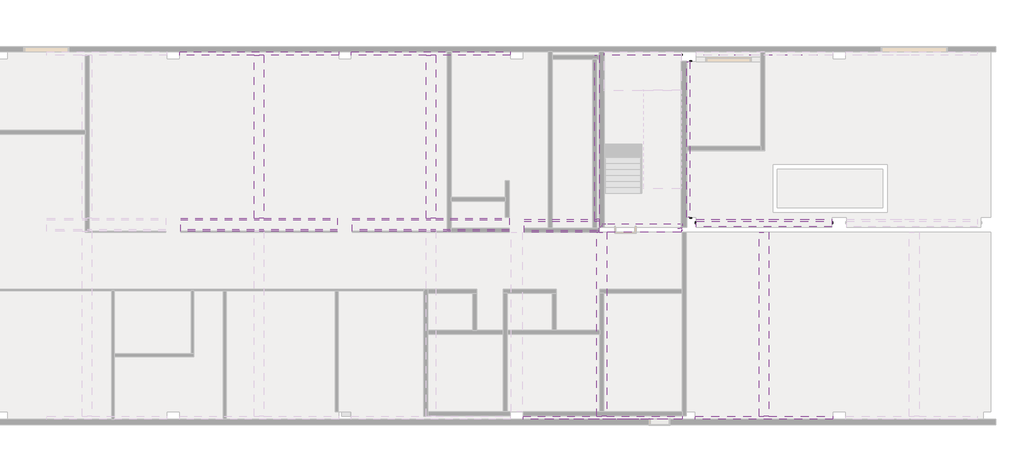
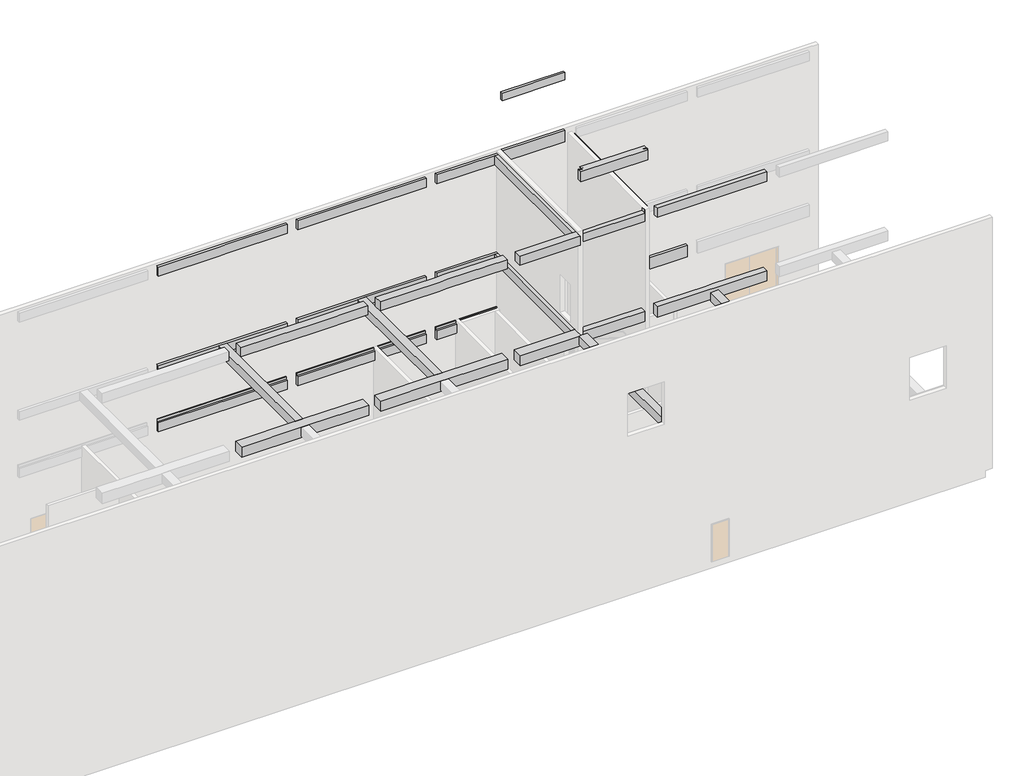
# One storey, part 4 of 5: 55 beams.
"""IFC4 building model written with IfcOpenShell, lengths in millimetres."""

from ifc_helpers import new_model, si_unit, frame, origin, place, context, project, spatial, polyline, outline, extrude, faceted_brep, element, save

model = new_model("IFC4")

# Units and contexts
model_context = context("Model", 3, world=origin())
ifc_project = project(units=[si_unit("LENGTHUNIT", "METRE", prefix="MILLI")], contexts=[model_context])

# Site, building, storey
site = spatial("IfcSite", under=ifc_project)
building = spatial("IfcBuilding", under=site)
storey = spatial("IfcBuildingStorey", under=building, Name="TOC", Elevation=149.9618634)

# Beams
placement = place(None, origin())
element("IfcBeam", 1, ObjectType="RC Beam_Rectangular : H_SB_AR_S16_UG_B500xH700_1G1", at=placement, inside=storey, context=model_context, shape_type="Brep", body=[
    faceted_brep([(61750.0, 799.5208589, -0.0381366), (61750.0, 9149.5208589, -0.0381366), (61750.0, 9149.5208589, -150.0381366), (61750.0, 9149.5208589, -550.0381366), (61750.0, 799.5208589, -550.0381366), (62250.0, 9149.5208589, -550.0381366), (62250.0, 799.5208589, -550.0381366), (62250.0, 9149.5208589, -0.0381366), (62250.0, 799.5208589, -0.0381366), (62250.0, 9149.5208589, -150.0381366)], [[[0, 1, 2, 3, 4]], [[3, 5, 6, 4]], [[7, 8, 6, 5, 9]], [[1, 0, 8, 7]], [[5, 3, 2, 1, 7, 9]], [[4, 6, 8, 0]]]),
])
element("IfcBeam", 2, ObjectType="RC Beam_Rectangular : H_SB_AR_S16_UG_B500xH700_1G1", at=placement, inside=storey, context=model_context, shape_type="Brep", body=[
    faceted_brep([(54700.0, 799.5208589, -0.0381366), (54700.0, 9149.5208589, -0.0381366), (54700.0, 9149.5208589, -150.0381366), (54700.0, 9149.5208589, -550.0381366), (54700.0, 799.5208589, -550.0381366), (54700.0, 799.5208589, -150.0381366), (55200.0, 799.5208589, -550.0381366), (54850.0, 9149.5208589, -550.0381366), (55200.0, 9149.5208589, -550.0381366), (55200.0, 9149.5208589, -0.0381366), (55200.0, 799.5208589, -0.0381366), (55200.0, 9149.5208589, -150.0381366)], [[[0, 1, 2, 3, 4, 5]], [[6, 4, 3, 7, 8]], [[9, 10, 6, 8, 11]], [[1, 0, 10, 9]], [[1, 9, 11, 8, 7, 3, 2]], [[4, 6, 10, 0, 5]]]),
])
element("IfcBeam", 3, ObjectType="RC Beam_Rectangular : H_SB_AR_S16_UG_B450xH700_1B2", at=placement, inside=storey, context=model_context, shape_type="SweptSolid", body=[
    extrude(outline(polyline([(57725.0, 599.5208589), (57275.0, 599.5208589), (57275.0, 9149.5208589), (57725.0, 9149.5208589), (57725.0, 599.5208589)])), frame((0.0, 0.0, -550.0381366), z_axis=(0.0, 0.0, 1.0), x_axis=(1.0, 0.0, 0.0)), (0.0, 0.0, 1.0), 550.0),
])
element("IfcBeam", 4, ObjectType="RC Beam_Rectangular : H_SB_AR_S16_UG_B450xH700_1B2", at=placement, inside=storey, context=model_context, shape_type="SweptSolid", body=[
    extrude(outline(polyline([(60225.0, 599.5208589), (59775.0, 599.5208589), (59775.0, 9149.5208589), (60225.0, 9149.5208589), (60225.0, 599.5208589)])), frame((0.0, 0.0, -550.0381366), z_axis=(0.0, 0.0, 1.0), x_axis=(1.0, 0.0, 0.0)), (0.0, 0.0, 1.0), 550.0),
])
element("IfcBeam", 5, ObjectType="RC Beam_Rectangular : H_SB_AR_S16_UG_B450xH700_1B1A", at=placement, inside=storey, context=model_context, shape_type="Brep", body=[
    faceted_brep([(51175.0, 599.5208589, -0.0381366), (51175.0, 599.5208589, -550.0381366), (51175.0, 9149.5208589, -550.0381366), (51175.0, 9149.5208589, -0.0381366), (50725.0, 599.5208589, -550.0381366), (50725.0, 9199.5208589, -550.0381366), (50725.0, 9799.5208589, -550.0381366), (50825.0, 9799.5208589, -550.0381366), (50825.0, 9149.5208589, -550.0381366), (50725.0, 599.5208589, -0.0381366), (50725.0, 9199.5208589, -0.0381366), (50725.0, 9799.5208589, -0.0381366), (50825.0, 9149.5208589, -0.0381366), (50825.0, 9799.5208589, -0.0381366)], [[[0, 1, 2, 3]], [[4, 5, 6, 7, 8, 2, 1]], [[6, 5, 4, 9, 10, 11]], [[4, 1, 0, 9]], [[0, 3, 12, 13, 11, 10, 9]], [[12, 8, 7, 13]], [[6, 11, 13, 7]], [[8, 12, 3, 2]]]),
])
element("IfcBeam", 6, ObjectType="RC Beam_Rectangular : H_SB_AR_S16_UG_B500xH700_1G3", at=placement, inside=storey, context=model_context, shape_type="SweptSolid", body=[
    extrude(outline(polyline([(-550.0381366, 55300.0), (-550.0381366, 61700.0), (-150.0381366, 61700.0), (-150.0381366, 61650.0), (-0.0381366, 61650.0), (-0.0381366, 55350.0), (-150.0381366, 55350.0), (-150.0381366, 55300.0), (-550.0381366, 55300.0)])), frame((0.0, 9549.5208589, 0.0), z_axis=(0.0, 1.0, 0.0), x_axis=(0.0, 0.0, 1.0)), (0.0, 0.0, 1.0), 100.0),
])
element("IfcBeam", 7, ObjectType="RC Beam_Rectangular : H_SB_AR_S16_UG_B600xH800_1G2", at=placement, inside=storey, context=model_context, shape_type="SweptSolid", body=[
    extrude(outline(polyline([(51225.0, 9799.5208589), (54650.0, 9799.5208589), (54650.0, 9549.5208589), (51225.0, 9549.5208589), (51225.0, 9799.5208589)])), frame((0.0, 0.0, -550.0381366), z_axis=(0.0, 0.0, 1.0), x_axis=(1.0, 0.0, 0.0)), (0.0, 0.0, 1.0), 500.0),
    extrude(outline(polyline([(-150.0381366, 47300.0), (-550.0381366, 47300.0), (-550.0381366, 48500.0), (-650.0381366, 48500.0), (-650.0381366, 49775.0), (-550.0381366, 49775.0), (-550.0381366, 50725.0), (-0.0381366, 50725.0), (-0.0381366, 47350.0), (-150.0381366, 47350.0), (-150.0381366, 47300.0)])), frame((0.0, 9199.5208589, 0.0), z_axis=(0.0, 1.0, 0.0), x_axis=(0.0, 0.0, 1.0)), (0.0, 0.0, 1.0), 600.0),
])
element("IfcBeam", 8, ObjectType="RC Beam_Rectangular : H_SB_AR_S16_UG_B600xH800_1G2", at=placement, inside=storey, context=model_context, shape_type="Brep", body=[
    faceted_brep([(39300.0, 9749.5208589, -550.0381366), (39300.0, 9749.5208589, -150.0381366), (39350.0, 9749.5208589, -150.0381366), (39350.0, 9749.5208589, -0.0381366), (42775.0, 9749.5208589, -0.0381366), (43225.0, 9749.5208589, -0.0381366), (46650.0, 9749.5208589, -0.0381366), (46650.0, 9749.5208589, -150.0381366), (46700.0, 9749.5208589, -150.0381366), (46700.0, 9749.5208589, -550.0381366), (45500.0, 9749.5208589, -550.0381366), (45500.0, 9749.5208589, -650.0381366), (40500.0, 9749.5208589, -650.0381366), (40500.0, 9749.5208589, -550.0381366), (40500.0, 9149.5208589, -650.0381366), (45500.0, 9149.5208589, -650.0381366), (38750.0, 9149.5208589, -550.0381366), (40500.0, 9149.5208589, -550.0381366), (45500.0, 9149.5208589, -550.0381366), (46750.0, 9149.5208589, -550.0381366), (47250.0, 9149.5208589, -550.0381366), (47250.0, 9149.5208589, -150.0381366), (46650.0, 9149.5208589, -150.0381366), (46650.0, 9149.5208589, -0.0381366), (43225.0, 9149.5208589, -0.0381366), (42775.0, 9149.5208589, -0.0381366), (39350.0, 9149.5208589, -0.0381366), (39350.0, 9149.5208589, -150.0381366), (38750.0, 9149.5208589, -150.0381366), (39300.0, 9199.5208589, -550.0381366), (39300.0, 9199.5208589, -150.0381366), (46700.0, 9199.5208589, -150.0381366), (46700.0, 9199.5208589, -550.0381366), (38750.0, 9199.5208589, -550.0381366), (46750.0, 9199.5208589, -550.0381366), (47250.0, 9199.5208589, -550.0381366), (38750.0, 9199.5208589, -150.0381366), (46750.0, 9199.5208589, -150.0381366), (47250.0, 9199.5208589, -150.0381366)], [[[0, 1, 2, 3, 4, 5, 6, 7, 8, 9, 10, 11, 12, 13]], [[14, 12, 11, 15]], [[16, 17, 14, 15, 18, 19, 20, 21, 22, 23, 24, 25, 26, 27, 28]], [[29, 30, 1, 0]], [[31, 32, 9, 8]], [[13, 17, 16, 33, 29, 0]], [[17, 13, 12, 14]], [[18, 10, 9, 32, 34, 35, 20, 19]], [[10, 18, 15, 11]], [[3, 26, 25, 24, 23, 6, 5, 4]], [[30, 29, 33, 36]], [[32, 31, 37, 38, 35, 34]], [[27, 2, 1, 30, 36, 28]], [[2, 27, 26, 3]], [[7, 22, 21, 38, 37, 31, 8]], [[22, 7, 6, 23]], [[36, 33, 16, 28]], [[20, 35, 38, 21]]]),
])
element("IfcBeam", 9, ObjectType="RC Beam_Rectangular : H_SB_AR_S16_UG_B600xH800_1G2", at=placement, inside=storey, context=model_context, shape_type="Brep", body=[
    faceted_brep([(38700.0, 9749.5208589, -150.0381366), (38700.0, 9749.5208589, -550.0381366), (37797.3745649, 9749.5208589, -550.0381366), (37797.3745649, 9749.5208589, -0.0381366), (38650.0, 9749.5208589, -0.0381366), (38650.0, 9749.5208589, -150.0381366), (37797.3745649, 9500.8571094, -550.0381366), (37797.3745649, 9500.8571094, -0.0381366), (38650.0, 9499.9097478, -0.0381366), (38650.0, 9499.9097478, -150.0381366), (38700.0, 9499.8541922, -150.0381366), (38700.0, 9499.8541922, -550.0381366)], [[[0, 1, 2, 3, 4, 5]], [[2, 6, 7, 3]], [[3, 7, 8, 4]], [[5, 9, 10, 0]], [[11, 10, 9, 8, 7, 6]], [[1, 0, 10, 11]], [[2, 1, 11, 6]], [[9, 5, 4, 8]]]),
    faceted_brep([(38749.6109568, 9149.5208589, -150.0381366), (38749.6109568, 9149.5208589, -550.0381366), (38750.0, 9149.5208589, -550.0381366), (38750.0, 9149.5208589, -150.0381366), (38749.6665123, 9199.5208589, -550.0381366), (38750.0, 9199.5208589, -550.0381366), (38749.6665123, 9199.5208589, -150.0381366), (38750.0, 9199.5208589, -150.0381366)], [[[0, 1, 2, 3]], [[1, 4, 5, 2]], [[4, 6, 7, 5]], [[6, 4, 1, 0]], [[3, 2, 5, 7]], [[6, 0, 3, 7]]]),
])
element("IfcBeam", 10, ObjectType="RC Beam_Rectangular : H_SB_AR_S16_UG_B450xH700_1B1", at=placement, inside=storey, context=model_context, shape_type="SweptSolid", body=[
    extrude(outline(polyline([(34775.0, 17399.5208589), (35225.0, 17399.5208589), (35225.0, 9749.5208589), (34775.0, 9749.5208589), (34775.0, 17399.5208589)])), frame((0.0, 0.0, -550.0381366), z_axis=(0.0, 0.0, 1.0), x_axis=(1.0, 0.0, 0.0)), (0.0, 0.0, 1.0), 550.0),
])
element("IfcBeam", 11, ObjectType="RC Beam_Rectangular : H_SB_AR_S16_UG_B450xH700_1B1", at=placement, inside=storey, context=model_context, shape_type="SweptSolid", body=[
    extrude(outline(polyline([(42775.0, 17399.5208589), (43225.0, 17399.5208589), (43225.0, 9749.5208589), (42775.0, 9749.5208589), (42775.0, 17399.5208589)])), frame((0.0, 0.0, -550.0381366), z_axis=(0.0, 0.0, 1.0), x_axis=(1.0, 0.0, 0.0)), (0.0, 0.0, 1.0), 550.0),
])
element("IfcBeam", 12, ObjectType="RC Beam_Rectangular : H_SB_AR_S16_UG_B500xH700_1G1", at=placement, inside=storey, context=model_context, shape_type="SweptSolid", body=[
    extrude(outline(polyline([(17199.5208589, -550.0381366), (9799.5208589, -550.0381366), (9799.5208589, -150.0381366), (9849.5208589, -150.0381366), (9849.5208589, -0.0381366), (17199.5208589, -0.0381366), (17199.5208589, -550.0381366)])), frame((46750.0, 0.0, 0.0), z_axis=(1.0, 0.0, 0.0), x_axis=(0.0, 1.0, 0.0)), (0.0, 0.0, 1.0), 500.0),
])
element("IfcBeam", 13, ObjectType="RC Beam_Rectangular : H_SB_AR_S16_UG_B500xH700_1G1", at=placement, inside=storey, context=model_context, shape_type="SweptSolid", body=[
    extrude(outline(polyline([(9799.5208589, -550.0381366), (9799.5208589, -150.0381366), (9849.5208589, -150.0381366), (9849.5208589, -0.0381366), (17199.5208589, -0.0381366), (17199.5208589, -550.0381366), (9799.5208589, -550.0381366)])), frame((38750.0, 0.0, 0.0), z_axis=(1.0, 0.0, 0.0), x_axis=(0.0, 1.0, 0.0)), (0.0, 0.0, 1.0), 500.0),
])
element("IfcBeam", 14, ObjectType="RC Beam_Rectangular : H_SB_AR_S16_UG_B500xH700_1G1", at=placement, inside=storey, context=model_context, shape_type="SweptSolid", body=[
    extrude(outline(polyline([(17149.5208589, -550.0381366), (9799.5208589, -550.0381366), (9799.5208589, -150.0381366), (9849.5208589, -150.0381366), (9849.5208589, -0.0381366), (17099.5208589, -0.0381366), (17099.5208589, -150.0381366), (17149.5208589, -150.0381366), (17149.5208589, -550.0381366)])), frame((55050.0, 0.0, 0.0), z_axis=(1.0, 0.0, 0.0), x_axis=(0.0, 1.0, 0.0)), (0.0, 0.0, 1.0), 100.0),
    extrude(outline(polyline([(54650.0, 17449.5208589), (54700.0, 17449.5208589), (54700.0, 17399.5208589), (54650.0, 17399.5208589), (54650.0, 17449.5208589)])), frame((0.0, 0.0, -550.0381366), z_axis=(0.0, 0.0, 1.0), x_axis=(1.0, 0.0, 0.0)), (0.0, 0.0, 1.0), 400.0),
])
element("IfcBeam", 15, ObjectType="RC Beam_Rectangular : H_SB_AR_S16_AG_B400xH700_3WG1", at=placement, inside=storey, context=model_context, shape_type="Brep", body=[
    faceted_brep([(31300.0, 17499.5208589, 5949.9618634), (38700.0, 17499.5208589, 5949.9618634), (38700.0, 17549.5208589, 5949.9618634), (31300.0, 17549.5208589, 5949.9618634), (31300.0, 17399.5208589, 5799.9618634), (31300.0, 17399.5208589, 5249.9618634), (34775.0, 17399.5208589, 5249.9618634), (35225.0, 17399.5208589, 5249.9618634), (38700.0, 17399.5208589, 5249.9618634), (38700.0, 17399.5208589, 5799.9618634), (35225.0, 17399.5208589, 5799.9618634), (34775.0, 17399.5208589, 5799.9618634), (31300.0, 17549.5208589, 5249.9618634), (38700.0, 17549.5208589, 5249.9618634), (31300.0, 17499.5208589, 5799.9618634), (38700.0, 17499.5208589, 5799.9618634)], [[[0, 1, 2, 3]], [[4, 5, 6, 7, 8, 9, 10, 11]], [[8, 7, 6, 5, 12, 13]], [[14, 4, 11, 10, 9, 15]], [[0, 14, 15, 1]], [[5, 4, 14, 0, 3, 12]], [[9, 8, 13, 2, 1, 15]], [[3, 2, 13, 12]]]),
])
element("IfcBeam", 16, ObjectType="RC Beam_Rectangular : H_SB_AR_S16_AG_B400xH700_3WG1", at=placement, inside=storey, context=model_context, shape_type="Brep", body=[
    faceted_brep([(39300.0, 17499.5208589, 5949.9618634), (46700.0, 17499.5208589, 5949.9618634), (46700.0, 17549.5208589, 5949.9618634), (39300.0, 17549.5208589, 5949.9618634), (39300.0, 17399.5208589, 5799.9618634), (39300.0, 17399.5208589, 5249.9618634), (42775.0, 17399.5208589, 5249.9618634), (43225.0, 17399.5208589, 5249.9618634), (46700.0, 17399.5208589, 5249.9618634), (46700.0, 17399.5208589, 5799.9618634), (43225.0, 17399.5208589, 5799.9618634), (42775.0, 17399.5208589, 5799.9618634), (39300.0, 17549.5208589, 5249.9618634), (46700.0, 17549.5208589, 5249.9618634), (39300.0, 17499.5208589, 5799.9618634), (46700.0, 17499.5208589, 5799.9618634)], [[[0, 1, 2, 3]], [[4, 5, 6, 7, 8, 9, 10, 11]], [[8, 7, 6, 5, 12, 13]], [[14, 4, 11, 10, 9, 15]], [[0, 14, 15, 1]], [[5, 4, 14, 0, 3, 12]], [[9, 8, 13, 2, 1, 15]], [[3, 2, 13, 12]]]),
])
element("IfcBeam", 17, ObjectType="RC Beam_Rectangular : H_SB_AR_S16_AG_B400xH700_3WG1", at=placement, inside=storey, context=model_context, shape_type="Brep", body=[
    faceted_brep([(51075.0, 17549.5208589, 5949.9618634), (51075.0, 17399.5208589, 5949.9618634), (54650.0, 17399.5208589, 5949.9618634), (54650.0, 17549.5208589, 5949.9618634), (51075.0, 17399.5208589, 5249.9618634), (54650.0, 17399.5208589, 5249.9618634), (51075.0, 17549.5208589, 5249.9618634), (54650.0, 17549.5208589, 5249.9618634)], [[[0, 1, 2, 3]], [[1, 4, 5, 2]], [[4, 6, 7, 5]], [[4, 1, 0, 6]], [[2, 5, 7, 3]], [[0, 3, 7, 6]]]),
    faceted_brep([(50825.0, 17399.5208589, 5249.9618634), (50825.0, 17549.5208589, 5249.9618634), (50825.0, 17549.5208589, 5949.9618634), (50825.0, 17499.5208589, 5949.9618634), (50825.0, 17499.5208589, 5799.9618634), (50825.0, 17399.5208589, 5799.9618634), (50625.0, 17399.5208589, 5799.9618634), (47300.0, 17399.5208589, 5799.9618634), (47300.0, 17399.5208589, 5249.9618634), (50625.0, 17399.5208589, 5249.9618634), (47300.0, 17499.5208589, 5799.9618634), (47300.0, 17499.5208589, 5949.9618634), (47300.0, 17549.5208589, 5949.9618634), (47300.0, 17549.5208589, 5249.9618634)], [[[0, 1, 2, 3, 4, 5]], [[0, 5, 6, 7, 8, 9]], [[5, 4, 10, 7, 6]], [[4, 3, 11, 10]], [[7, 10, 11, 12, 13, 8]], [[12, 2, 1, 13]], [[3, 2, 12, 11]], [[1, 0, 9, 8, 13]]]),
])
element("IfcBeam", 18, ObjectType="RC Beam_Rectangular : H_SB_AR_S16_AG_B400xH700_3WG1", at=placement, inside=storey, context=model_context, shape_type="SweptSolid", body=[
    extrude(outline(polyline([(61700.0, 17399.5208589), (55350.0, 17399.5208589), (55350.0, 17549.5208589), (61700.0, 17549.5208589), (61700.0, 17399.5208589)])), frame((0.0, 0.0, 5249.9618634), z_axis=(0.0, 0.0, 1.0), x_axis=(1.0, 0.0, 0.0)), (0.0, 0.0, 1.0), 700.0),
])
element("IfcBeam", 19, ObjectType="RC Beam_Rectangular : H_SB_AR_S16_AG_B400xH700_3WG1", at=placement, inside=storey, context=model_context, shape_type="Brep", body=[
    faceted_brep([(54700.0, 499.5208589, 5949.9618634), (50950.0, 499.5208589, 5949.9618634), (47300.0, 499.5208589, 5949.9618634), (47300.0, 449.5208589, 5949.9618634), (54700.0, 449.5208589, 5949.9618634), (54700.0, 599.5208589, 5249.9618634), (54700.0, 449.5208589, 5249.9618634), (47300.0, 449.5208589, 5249.9618634), (47300.0, 599.5208589, 5249.9618634), (50725.0, 599.5208589, 5249.9618634), (51175.0, 599.5208589, 5249.9618634), (54700.0, 599.5208589, 5799.9618634), (47300.0, 599.5208589, 5799.9618634), (50725.0, 599.5208589, 5799.9618634), (51175.0, 599.5208589, 5799.9618634), (50950.0, 499.5208589, 5799.9618634), (54700.0, 499.5208589, 5799.9618634), (47300.0, 499.5208589, 5799.9618634)], [[[0, 1, 2, 3, 4]], [[5, 6, 7, 8, 9, 10]], [[11, 5, 10, 9, 8, 12, 13, 14]], [[6, 4, 3, 7]], [[15, 16, 11, 14, 13, 12, 17]], [[15, 1, 0, 16]], [[1, 15, 17, 2]], [[0, 4, 6, 5, 11, 16]], [[3, 2, 17, 12, 8, 7]]]),
])
element("IfcBeam", 20, ObjectType="RC Beam_Rectangular : H_SB_AR_S16_AG_B400xH700_3WG1", at=placement, inside=storey, context=model_context, shape_type="Brep", body=[
    faceted_brep([(61700.0, 449.5208589, 5949.9618634), (61700.0, 499.5208589, 5949.9618634), (55300.0, 499.5208589, 5949.9618634), (55300.0, 449.5208589, 5949.9618634), (61700.0, 599.5208589, 5249.9618634), (61700.0, 449.5208589, 5249.9618634), (55300.0, 449.5208589, 5249.9618634), (55300.0, 599.5208589, 5249.9618634), (58275.0, 599.5208589, 5249.9618634), (58725.0, 599.5208589, 5249.9618634), (61700.0, 599.5208589, 5799.9618634), (55300.0, 599.5208589, 5799.9618634), (58275.0, 599.5208589, 5799.9618634), (58725.0, 599.5208589, 5799.9618634), (61700.0, 499.5208589, 5799.9618634), (55300.0, 499.5208589, 5799.9618634)], [[[0, 1, 2, 3]], [[4, 5, 6, 7, 8, 9]], [[10, 4, 9, 8, 7, 11, 12, 13]], [[5, 0, 3, 6]], [[14, 10, 13, 12, 11, 15]], [[1, 14, 15, 2]], [[1, 0, 5, 4, 10, 14]], [[3, 2, 15, 11, 7, 6]]]),
])
element("IfcBeam", 21, ObjectType="RC Beam_Rectangular : H_SB_AR_S16_AG_B600xH800_3G2", at=placement, inside=storey, context=model_context, shape_type="Brep", body=[
    faceted_brep([(31350.0, 9199.5208589, 5149.9618634), (38650.0, 9199.5208589, 5149.9618634), (38650.0, 9199.5208589, 5799.9618634), (35235.0, 9199.5208589, 5799.9618634), (34785.0, 9199.5208589, 5799.9618634), (31350.0, 9199.5208589, 5799.9618634), (31350.0, 9799.5208589, 5149.9618634), (38650.0, 9799.5208589, 5149.9618634), (31350.0, 9799.5208589, 5799.9618634), (34775.0, 9799.5208589, 5799.9618634), (35225.0, 9799.5208589, 5799.9618634), (38650.0, 9799.5208589, 5799.9618634)], [[[0, 1, 2, 3, 4, 5]], [[1, 0, 6, 7]], [[7, 6, 8, 9, 10, 11]], [[5, 4, 3, 2, 11, 10, 9, 8]], [[6, 0, 5, 8]], [[1, 7, 11, 2]]]),
])
element("IfcBeam", 22, ObjectType="RC Beam_Rectangular : H_SB_AR_S16_AG_B600xH800_3G2", at=placement, inside=storey, context=model_context, shape_type="Brep", body=[
    faceted_brep([(39350.0, 9199.5208589, 5149.9618634), (46650.0, 9199.5208589, 5149.9618634), (46650.0, 9199.5208589, 5799.9618634), (43235.0, 9199.5208589, 5799.9618634), (42785.0, 9199.5208589, 5799.9618634), (39350.0, 9199.5208589, 5799.9618634), (39350.0, 9799.5208589, 5149.9618634), (46650.0, 9799.5208589, 5149.9618634), (39350.0, 9799.5208589, 5799.9618634), (42775.0, 9799.5208589, 5799.9618634), (43225.0, 9799.5208589, 5799.9618634), (46650.0, 9799.5208589, 5799.9618634)], [[[0, 1, 2, 3, 4, 5]], [[1, 0, 6, 7]], [[7, 6, 8, 9, 10, 11]], [[5, 4, 3, 2, 11, 10, 9, 8]], [[6, 0, 5, 8]], [[1, 7, 11, 2]]]),
])
element("IfcBeam", 23, ObjectType="RC Beam_Rectangular : H_SB_AR_S16_AG_B600xH800_3WG2", at=placement, inside=storey, context=model_context, shape_type="Brep", body=[
    faceted_brep([(50825.0, 9149.5208589, 5149.9618634), (50825.0, 9149.5208589, 5799.9618634), (50725.0, 9149.5208589, 5799.9618634), (47350.0, 9149.5208589, 5799.9618634), (47350.0, 9149.5208589, 5149.9618634), (50825.0, 9749.5208589, 5149.9618634), (50825.0, 9749.5208589, 5249.9618634), (50825.0, 9749.5208589, 5799.9618634), (50625.0, 9749.5208589, 5799.9618634), (47350.0, 9749.5208589, 5799.9618634), (47350.0, 9749.5208589, 5149.9618634)], [[[0, 1, 2, 3, 4]], [[0, 5, 6, 7, 1]], [[3, 2, 1, 7, 8, 9]], [[10, 4, 3, 9]], [[5, 0, 4, 10]], [[5, 10, 9, 8, 7, 6]]]),
    faceted_brep([(54650.0, 9399.5208589, 5149.9618634), (54650.0, 9749.5208589, 5149.9618634), (54650.0, 9749.5208589, 5749.9618634), (54650.0, 9399.5208589, 5749.9618634), (51075.0, 9399.5208589, 5749.9618634), (51075.0, 9749.5208589, 5749.9618634), (51075.0, 9749.5208589, 5149.9618634), (51075.0, 9399.5208589, 5149.9618634)], [[[0, 1, 2, 3]], [[4, 5, 6, 7]], [[5, 4, 3, 2]], [[1, 0, 7, 6]], [[1, 6, 5, 2]], [[7, 0, 3, 4]]]),
])
element("IfcBeam", 24, ObjectType="RC Beam_Rectangular : H_SB_AR_S16_AG_B600xH800_3WG2", at=placement, inside=storey, context=model_context, shape_type="SweptSolid", body=[
    extrude(outline(polyline([(55350.0, 9399.5208589), (55350.0, 9749.5208589), (61650.0, 9749.5208589), (61650.0, 9399.5208589), (55350.0, 9399.5208589)])), frame((0.0, 0.0, 5149.9618634), z_axis=(0.0, 0.0, 1.0), x_axis=(1.0, 0.0, 0.0)), (0.0, 0.0, 1.0), 800.0),
])
element("IfcBeam", 25, ObjectType="RC Beam_Rectangular : H_SB_AR_S16_AG_B400xH700_3WG3", at=placement, inside=storey, context=model_context, shape_type="SweptSolid", body=[
    extrude(outline(polyline([(55050.0, 9849.5208589), (54900.0, 9849.5208589), (54900.0, 17099.5208589), (55050.0, 17099.5208589), (55050.0, 9849.5208589)])), frame((0.0, 0.0, 5249.9618634), z_axis=(0.0, 0.0, 1.0), x_axis=(1.0, 0.0, 0.0)), (0.0, 0.0, 1.0), 700.0),
])
element("IfcBeam", 26, ObjectType="RC Beam_Rectangular : H_SB_AR_S16_AG_B450xH700_2WB1", at=placement, inside=storey, context=model_context, shape_type="SweptSolid", body=[
    extrude(outline(polyline([(50825.0, 9749.5208589), (50625.0, 9749.5208589), (50625.0, 17399.5208589), (50825.0, 17399.5208589), (50825.0, 9749.5208589)])), frame((0.0, 0.0, 5249.9618634), z_axis=(0.0, 0.0, 1.0), x_axis=(1.0, 0.0, 0.0)), (0.0, 0.0, 1.0), 550.0),
])
element("IfcBeam", 27, ObjectType="RC Beam_Rectangular : H_SB_AR_S16_AG_B450xH700_3B1", at=placement, inside=storey, context=model_context, shape_type="SweptSolid", body=[
    extrude(outline(polyline([(58275.0, 9149.5208589), (58725.0, 9149.5208589), (58725.0, 599.5208589), (58275.0, 599.5208589), (58275.0, 9149.5208589)])), frame((0.0, 0.0, 5249.9618634), z_axis=(0.0, 0.0, 1.0), x_axis=(1.0, 0.0, 0.0)), (0.0, 0.0, 1.0), 550.0),
])
element("IfcBeam", 28, ObjectType="RC Beam_Rectangular : H_SB_AR_S16_AG_B400xH700_3WG1", at=placement, inside=storey, context=model_context, shape_type="Brep", body=[
    faceted_brep([(31300.0, 17399.5208589, 9269.9618634), (31300.0, 17399.5208589, 8749.9618634), (34775.0, 17399.5208589, 8749.9618634), (35225.0, 17399.5208589, 8749.9618634), (38700.0, 17399.5208589, 8749.9618634), (38700.0, 17399.5208589, 9269.9618634), (35225.0, 17399.5208589, 9269.9618634), (34775.0, 17399.5208589, 9269.9618634), (31300.0, 17549.5208589, 8749.9618634), (38700.0, 17549.5208589, 8749.9618634), (31300.0, 17549.5208589, 9269.9618634), (38700.0, 17549.5208589, 9269.9618634)], [[[0, 1, 2, 3, 4, 5, 6, 7]], [[4, 3, 2, 1, 8, 9]], [[10, 0, 7, 6, 5, 11]], [[1, 0, 10, 8]], [[5, 4, 9, 11]], [[9, 8, 10, 11]]]),
])
element("IfcBeam", 29, ObjectType="RC Beam_Rectangular : H_SB_AR_S16_AG_B400xH700_3WG1", at=placement, inside=storey, context=model_context, shape_type="Brep", body=[
    faceted_brep([(39300.0, 17399.5208589, 9269.9618634), (39300.0, 17399.5208589, 8749.9618634), (42775.0, 17399.5208589, 8749.9618634), (43225.0, 17399.5208589, 8749.9618634), (46700.0, 17399.5208589, 8749.9618634), (46700.0, 17399.5208589, 9269.9618634), (43225.0, 17399.5208589, 9269.9618634), (42775.0, 17399.5208589, 9269.9618634), (39300.0, 17549.5208589, 8749.9618634), (46700.0, 17549.5208589, 8749.9618634), (39300.0, 17549.5208589, 9269.9618634), (46700.0, 17549.5208589, 9269.9618634)], [[[0, 1, 2, 3, 4, 5, 6, 7]], [[4, 3, 2, 1, 8, 9]], [[10, 0, 7, 6, 5, 11]], [[1, 0, 10, 8]], [[5, 4, 9, 11]], [[9, 8, 10, 11]]]),
])
element("IfcBeam", 30, ObjectType="RC Beam_Rectangular : H_SB_AR_S16_AG_B400xH700_3WG1", at=placement, inside=storey, context=model_context, shape_type="Brep", body=[
    faceted_brep([(51075.0, 17549.5208589, 9449.9618634), (51075.0, 17399.5208589, 9449.9618634), (54650.0, 17399.5208589, 9449.9618634), (54650.0, 17549.5208589, 9449.9618634), (51075.0, 17399.5208589, 9269.9618634), (51075.0, 17399.5208589, 8749.9618634), (54650.0, 17399.5208589, 8749.9618634), (51075.0, 17549.5208589, 8749.9618634), (54650.0, 17549.5208589, 8749.9618634), (51075.0, 17549.5208589, 9269.9618634)], [[[0, 1, 2, 3]], [[1, 4, 5, 6, 2]], [[5, 7, 8, 6]], [[7, 5, 4, 1, 0, 9]], [[2, 6, 8, 3]], [[0, 3, 8, 7, 9]]]),
    faceted_brep([(50825.0, 17399.5208589, 8749.9618634), (50825.0, 17549.5208589, 8749.9618634), (50825.0, 17549.5208589, 9269.9618634), (50825.0, 17399.5208589, 9269.9618634), (50625.0, 17399.5208589, 9269.9618634), (47300.0, 17399.5208589, 9269.9618634), (47300.0, 17399.5208589, 8749.9618634), (50625.0, 17399.5208589, 8749.9618634), (47300.0, 17549.5208589, 9269.9618634), (47300.0, 17549.5208589, 8749.9618634)], [[[0, 1, 2, 3]], [[0, 3, 4, 5, 6, 7]], [[3, 2, 8, 5, 4]], [[5, 8, 9, 6]], [[1, 9, 8, 2]], [[1, 0, 7, 6, 9]]]),
])
element("IfcBeam", 31, ObjectType="RC Beam_Rectangular : H_SB_AR_S16_AG_B400xH700_3WG1", at=placement, inside=storey, context=model_context, shape_type="Brep", body=[
    faceted_brep([(54700.0, 599.5208589, 8749.9618634), (54700.0, 449.5208589, 8749.9618634), (47300.0, 449.5208589, 8749.9618634), (47300.0, 599.5208589, 8749.9618634), (50725.0, 599.5208589, 8749.9618634), (51175.0, 599.5208589, 8749.9618634), (54700.0, 599.5208589, 9269.9618634), (47300.0, 599.5208589, 9269.9618634), (50725.0, 599.5208589, 9269.9618634), (51175.0, 599.5208589, 9269.9618634), (54700.0, 449.5208589, 9269.9618634), (50825.0, 449.5208589, 9269.9618634), (47300.0, 449.5208589, 9269.9618634)], [[[0, 1, 2, 3, 4, 5]], [[6, 0, 5, 4, 3, 7, 8, 9]], [[1, 10, 11, 12, 2]], [[10, 6, 9, 8, 7, 12, 11]], [[1, 0, 6, 10]], [[3, 2, 12, 7]]]),
])
element("IfcBeam", 32, ObjectType="RC Beam_Rectangular : H_SB_AR_S16_AG_B400xH700_3WG1", at=placement, inside=storey, context=model_context, shape_type="Brep", body=[
    faceted_brep([(61700.0, 599.5208589, 8749.9618634), (61700.0, 449.5208589, 8749.9618634), (55300.0, 449.5208589, 8749.9618634), (55300.0, 599.5208589, 8749.9618634), (58275.0, 599.5208589, 8749.9618634), (58725.0, 599.5208589, 8749.9618634), (61700.0, 599.5208589, 9269.9618634), (55300.0, 599.5208589, 9269.9618634), (58275.0, 599.5208589, 9269.9618634), (58725.0, 599.5208589, 9269.9618634), (61700.0, 449.5208589, 9269.9618634), (55300.0, 449.5208589, 9269.9618634)], [[[0, 1, 2, 3, 4, 5]], [[6, 0, 5, 4, 3, 7, 8, 9]], [[1, 10, 11, 2]], [[10, 6, 9, 8, 7, 11]], [[1, 0, 6, 10]], [[3, 2, 11, 7]]]),
])
element("IfcBeam", 33, ObjectType="RC Beam_Rectangular : H_SB_AR_S16_AG_B600xH800_3G2", at=placement, inside=storey, context=model_context, shape_type="Brep", body=[
    faceted_brep([(31350.0, 9199.5208589, 8649.9618634), (38650.0, 9199.5208589, 8649.9618634), (38650.0, 9199.5208589, 9269.9618634), (35225.0, 9199.5208589, 9269.9618634), (34775.0, 9199.5208589, 9269.9618634), (31350.0, 9199.5208589, 9269.9618634), (31350.0, 9799.5208589, 8649.9618634), (38650.0, 9799.5208589, 8649.9618634), (31350.0, 9799.5208589, 9269.9618634), (34775.0, 9799.5208589, 9269.9618634), (35225.0, 9799.5208589, 9269.9618634), (38650.0, 9799.5208589, 9269.9618634)], [[[0, 1, 2, 3, 4, 5]], [[1, 0, 6, 7]], [[7, 6, 8, 9, 10, 11]], [[5, 4, 3, 2, 11, 10, 9, 8]], [[6, 0, 5, 8]], [[1, 7, 11, 2]]]),
])
element("IfcBeam", 34, ObjectType="RC Beam_Rectangular : H_SB_AR_S16_AG_B600xH800_3G2", at=placement, inside=storey, context=model_context, shape_type="Brep", body=[
    faceted_brep([(39350.0, 9199.5208589, 8649.9618634), (46650.0, 9199.5208589, 8649.9618634), (46650.0, 9199.5208589, 9269.9618634), (43225.0, 9199.5208589, 9269.9618634), (42775.0, 9199.5208589, 9269.9618634), (39350.0, 9199.5208589, 9269.9618634), (39350.0, 9799.5208589, 8649.9618634), (46650.0, 9799.5208589, 8649.9618634), (39350.0, 9799.5208589, 9269.9618634), (42775.0, 9799.5208589, 9269.9618634), (43225.0, 9799.5208589, 9269.9618634), (46650.0, 9799.5208589, 9269.9618634)], [[[0, 1, 2, 3, 4, 5]], [[1, 0, 6, 7]], [[7, 6, 8, 9, 10, 11]], [[5, 4, 3, 2, 11, 10, 9, 8]], [[6, 0, 5, 8]], [[1, 7, 11, 2]]]),
])
element("IfcBeam", 35, ObjectType="RC Beam_Rectangular : H_SB_AR_S16_AG_B600xH800_3WG2", at=placement, inside=storey, context=model_context, shape_type="Brep", body=[
    faceted_brep([(50825.0, 9149.5208589, 8649.9618634), (50825.0, 9149.5208589, 9269.9618634), (50725.0, 9149.5208589, 9269.9618634), (47350.0, 9149.5208589, 9269.9618634), (47350.0, 9149.5208589, 8649.9618634), (50825.0, 9749.5208589, 8649.9618634), (50825.0, 9749.5208589, 8749.9618634), (50825.0, 9749.5208589, 9269.9618634), (50625.0, 9749.5208589, 9269.9618634), (47350.0, 9749.5208589, 9269.9618634), (47350.0, 9749.5208589, 8649.9618634)], [[[0, 1, 2, 3, 4]], [[0, 5, 6, 7, 1]], [[3, 2, 1, 7, 8, 9]], [[10, 4, 3, 9]], [[5, 0, 4, 10]], [[5, 10, 9, 8, 7, 6]]]),
    faceted_brep([(54650.0, 9399.5208589, 8649.9618634), (54650.0, 9749.5208589, 8649.9618634), (54650.0, 9749.5208589, 9249.9618634), (54650.0, 9399.5208589, 9249.9618634), (51075.0, 9399.5208589, 9249.9618634), (51075.0, 9749.5208589, 9249.9618634), (51075.0, 9749.5208589, 8649.9618634), (51075.0, 9399.5208589, 8649.9618634)], [[[0, 1, 2, 3]], [[4, 5, 6, 7]], [[5, 4, 3, 2]], [[1, 0, 7, 6]], [[1, 6, 5, 2]], [[7, 0, 3, 4]]]),
])
element("IfcBeam", 36, ObjectType="RC Beam_Rectangular : H_SB_AR_S16_AG_B600xH800_3WG2", at=placement, inside=storey, context=model_context, shape_type="Brep", body=[
    faceted_brep([(55350.0, 9399.5208589, 8649.9618634), (55350.0, 9749.5208589, 8649.9618634), (61650.0, 9749.5208589, 8649.9618634), (61650.0, 9399.5208589, 8649.9618634), (55350.0, 9749.5208589, 9269.9618634), (58275.0, 9749.5208589, 9269.9618634), (58725.0, 9749.5208589, 9269.9618634), (61650.0, 9749.5208589, 9269.9618634), (55350.0, 9399.5208589, 9269.9618634), (61650.0, 9399.5208589, 9269.9618634)], [[[0, 1, 2, 3]], [[1, 4, 5, 6, 7, 2]], [[8, 0, 3, 9]], [[4, 8, 9, 7, 6, 5]], [[1, 0, 8, 4]], [[3, 2, 7, 9]]]),
])
element("IfcBeam", 37, ObjectType="RC Beam_Rectangular : H_SB_AR_S16_AG_B400xH700_3WG3", at=placement, inside=storey, context=model_context, shape_type="SweptSolid", body=[
    extrude(outline(polyline([(54900.0, 17099.5208589), (55050.0, 17099.5208589), (55050.0, 9849.5208589), (54900.0, 9849.5208589), (54900.0, 17099.5208589)])), frame((0.0, 0.0, 8749.9618634), z_axis=(0.0, 0.0, 1.0), x_axis=(1.0, 0.0, 0.0)), (0.0, 0.0, 1.0), 520.0),
])
element("IfcBeam", 38, ObjectType="RC Beam_Rectangular : H_SB_AR_S16_AG_B450xH700_3WB1", at=placement, inside=storey, context=model_context, shape_type="SweptSolid", body=[
    extrude(outline(polyline([(50625.0, 9749.5208589), (50625.0, 17399.5208589), (50825.0, 17399.5208589), (50825.0, 9749.5208589), (50625.0, 9749.5208589)])), frame((0.0, 0.0, 8749.9618634), z_axis=(0.0, 0.0, 1.0), x_axis=(1.0, 0.0, 0.0)), (0.0, 0.0, 1.0), 520.0),
])
element("IfcBeam", 39, ObjectType="RC Beam_Rectangular : H_SB_AR_S16_AG_B450xH700_3B1", at=placement, inside=storey, context=model_context, shape_type="SweptSolid", body=[
    extrude(outline(polyline([(34775.0, 17399.5208589), (35225.0, 17399.5208589), (35225.0, 9799.5208589), (34775.0, 9799.5208589), (34775.0, 17399.5208589)])), frame((0.0, 0.0, 8749.9618634), z_axis=(0.0, 0.0, 1.0), x_axis=(1.0, 0.0, 0.0)), (0.0, 0.0, 1.0), 520.0),
])
element("IfcBeam", 40, ObjectType="RC Beam_Rectangular : H_SB_AR_S16_AG_B450xH700_3B1", at=placement, inside=storey, context=model_context, shape_type="SweptSolid", body=[
    extrude(outline(polyline([(42775.0, 17399.5208589), (43225.0, 17399.5208589), (43225.0, 9799.5208589), (42775.0, 9799.5208589), (42775.0, 17399.5208589)])), frame((0.0, 0.0, 8749.9618634), z_axis=(0.0, 0.0, 1.0), x_axis=(1.0, 0.0, 0.0)), (0.0, 0.0, 1.0), 520.0),
])
element("IfcBeam", 41, ObjectType="RC Beam_Rectangular : H_SB_AR_S16_AG_B450xH700_3B1A", at=placement, inside=storey, context=model_context, shape_type="Brep", body=[
    faceted_brep([(50725.0, 9149.5208589, 8749.9618634), (50725.0, 599.5208589, 8749.9618634), (50725.0, 599.5208589, 9269.9618634), (50725.0, 9149.5208589, 9269.9618634), (51175.0, 9149.5208589, 8749.9618634), (51175.0, 599.5208589, 8749.9618634), (51175.0, 9149.5208589, 9269.9618634), (51175.0, 599.5208589, 9269.9618634), (50825.0, 9149.5208589, 9269.9618634)], [[[0, 1, 2, 3]], [[4, 5, 1, 0]], [[5, 4, 6, 7]], [[4, 0, 3, 8, 6]], [[1, 5, 7, 2]], [[3, 2, 7, 6, 8]]]),
])
element("IfcBeam", 42, ObjectType="RC Beam_Rectangular : H_SB_AR_S16_AG_B450xH700_3B1A", at=placement, inside=storey, context=model_context, shape_type="SweptSolid", body=[
    extrude(outline(polyline([(58275.0, 9149.5208589), (58725.0, 9149.5208589), (58725.0, 599.5208589), (58275.0, 599.5208589), (58275.0, 9149.5208589)])), frame((0.0, 0.0, 8749.9618634), z_axis=(0.0, 0.0, 1.0), x_axis=(1.0, 0.0, 0.0)), (0.0, 0.0, 1.0), 520.0),
])
element("IfcBeam", 43, ObjectType="RC Beam_Rectangular : H_SB_AR_S16_AG_B400xH700_RWG1", at=placement, inside=storey, context=model_context, shape_type="Brep", body=[
    faceted_brep([(31300.0, 17399.5208589, 15259.9618634), (31300.0, 17399.5208589, 14709.9618634), (34775.0, 17399.5208589, 14709.9618634), (35225.0, 17399.5208589, 14709.9618634), (38700.0, 17399.5208589, 14709.9618634), (38700.0, 17399.5208589, 15259.9618634), (35225.0, 17399.5208589, 15259.9618634), (34775.0, 17399.5208589, 15259.9618634), (31300.0, 17549.5208589, 14709.9618634), (38700.0, 17549.5208589, 14709.9618634), (31300.0, 17549.5208589, 15259.9618634), (38700.0, 17549.5208589, 15259.9618634)], [[[0, 1, 2, 3, 4, 5, 6, 7]], [[4, 3, 2, 1, 8, 9]], [[10, 0, 7, 6, 5, 11]], [[1, 0, 10, 8]], [[5, 4, 9, 11]], [[9, 8, 10, 11]]]),
])
element("IfcBeam", 44, ObjectType="RC Beam_Rectangular : H_SB_AR_S16_AG_B400xH700_RWG1", at=placement, inside=storey, context=model_context, shape_type="Brep", body=[
    faceted_brep([(39300.0, 17399.5208589, 15259.9618634), (39300.0, 17399.5208589, 14709.9618634), (42775.0, 17399.5208589, 14709.9618634), (43225.0, 17399.5208589, 14709.9618634), (46700.0, 17399.5208589, 14709.9618634), (46700.0, 17399.5208589, 15259.9618634), (43225.0, 17399.5208589, 15259.9618634), (42775.0, 17399.5208589, 15259.9618634), (39300.0, 17549.5208589, 14709.9618634), (46700.0, 17549.5208589, 14709.9618634), (39300.0, 17549.5208589, 15259.9618634), (46700.0, 17549.5208589, 15259.9618634)], [[[0, 1, 2, 3, 4, 5, 6, 7]], [[4, 3, 2, 1, 8, 9]], [[10, 0, 7, 6, 5, 11]], [[1, 0, 10, 8]], [[5, 4, 9, 11]], [[9, 8, 10, 11]]]),
])
element("IfcBeam", 45, ObjectType="RC Beam_Rectangular : H_SB_AR_S16_AG_B400xH700_RWG1", at=placement, inside=storey, context=model_context, shape_type="Brep", body=[
    faceted_brep([(51075.0, 17549.5208589, 15409.9618634), (51075.0, 17399.5208589, 15409.9618634), (54650.0, 17399.5208589, 15409.9618634), (54650.0, 17549.5208589, 15409.9618634), (51075.0, 17399.5208589, 15259.9618634), (51075.0, 17399.5208589, 14709.9618634), (54650.0, 17399.5208589, 14709.9618634), (51075.0, 17549.5208589, 14709.9618634), (54650.0, 17549.5208589, 14709.9618634), (51075.0, 17549.5208589, 15259.9618634), (54650.0, 17549.5208589, 15259.9618634)], [[[0, 1, 2, 3]], [[1, 4, 5, 6, 2]], [[5, 7, 8, 6]], [[7, 5, 4, 1, 0, 9]], [[2, 6, 8, 10, 3]], [[0, 3, 10, 8, 7, 9]]]),
    faceted_brep([(50825.0, 17399.5208589, 14709.9618634), (50825.0, 17549.5208589, 14709.9618634), (50825.0, 17549.5208589, 15259.9618634), (50825.0, 17399.5208589, 15259.9618634), (50625.0, 17399.5208589, 15259.9618634), (47300.0, 17399.5208589, 15259.9618634), (47300.0, 17399.5208589, 14709.9618634), (50625.0, 17399.5208589, 14709.9618634), (47300.0, 17549.5208589, 15259.9618634), (47300.0, 17549.5208589, 14709.9618634)], [[[0, 1, 2, 3]], [[0, 3, 4, 5, 6, 7]], [[3, 2, 8, 5, 4]], [[5, 8, 9, 6]], [[1, 9, 8, 2]], [[1, 0, 7, 6, 9]]]),
])
element("IfcBeam", 46, ObjectType="RC Beam_Rectangular : H_SB_AR_S16_AG_B400xH700_RWG1", at=placement, inside=storey, context=model_context, shape_type="Brep", body=[
    faceted_brep([(54700.0, 599.5208589, 14709.9618634), (54700.0, 449.5208589, 14709.9618634), (47300.0, 449.5208589, 14709.9618634), (47300.0, 599.5208589, 14709.9618634), (50725.0, 599.5208589, 14709.9618634), (51175.0, 599.5208589, 14709.9618634), (54700.0, 599.5208589, 15259.9618634), (47300.0, 599.5208589, 15259.9618634), (50725.0, 599.5208589, 15259.9618634), (51175.0, 599.5208589, 15259.9618634), (54700.0, 449.5208589, 15259.9618634), (50825.0, 449.5208589, 15259.9618634), (47300.0, 449.5208589, 15259.9618634)], [[[0, 1, 2, 3, 4, 5]], [[6, 0, 5, 4, 3, 7, 8, 9]], [[1, 10, 11, 12, 2]], [[10, 6, 9, 8, 7, 12, 11]], [[1, 0, 6, 10]], [[3, 2, 12, 7]]]),
])
element("IfcBeam", 47, ObjectType="RC Beam_Rectangular : H_SB_AR_S16_AG_B400xH700_RWG1", at=placement, inside=storey, context=model_context, shape_type="Brep", body=[
    faceted_brep([(61700.0, 599.5208589, 14709.9618634), (61700.0, 449.5208589, 14709.9618634), (55300.0, 449.5208589, 14709.9618634), (55300.0, 599.5208589, 14709.9618634), (58275.0, 599.5208589, 14709.9618634), (58725.0, 599.5208589, 14709.9618634), (61700.0, 599.5208589, 15259.9618634), (55300.0, 599.5208589, 15259.9618634), (58275.0, 599.5208589, 15259.9618634), (58725.0, 599.5208589, 15259.9618634), (61700.0, 449.5208589, 15259.9618634), (55300.0, 449.5208589, 15259.9618634)], [[[0, 1, 2, 3, 4, 5]], [[6, 0, 5, 4, 3, 7, 8, 9]], [[1, 10, 11, 2]], [[10, 6, 9, 8, 7, 11]], [[1, 0, 6, 10]], [[3, 2, 11, 7]]]),
])
element("IfcBeam", 48, ObjectType="RC Beam_Rectangular : H_SB_AR_S16_AG_B450xH700_RWG3", at=placement, inside=storey, context=model_context, shape_type="Brep", body=[
    faceted_brep([(55350.0, 9674.5208589, 14709.9618634), (55350.0, 9674.5208589, 15259.9618634), (58275.0, 9674.5208589, 15259.9618634), (58725.0, 9674.5208589, 15259.9618634), (61650.0, 9674.5208589, 15259.9618634), (61650.0, 9674.5208589, 14709.9618634), (58725.0, 9674.5208589, 14709.9618634), (58275.0, 9674.5208589, 14709.9618634), (55350.0, 9399.5208589, 14709.9618634), (61650.0, 9399.5208589, 14709.9618634), (55350.0, 9399.5208589, 15259.9618634), (61650.0, 9399.5208589, 15259.9618634)], [[[0, 1, 2, 3, 4, 5, 6, 7]], [[8, 0, 7, 6, 5, 9]], [[10, 8, 9, 11]], [[1, 10, 11, 4, 3, 2]], [[1, 0, 8, 10]], [[5, 4, 11, 9]]]),
])
element("IfcBeam", 49, ObjectType="RC Beam_Rectangular : H_SB_AR_S16_AG_B450xH700_RWG3", at=placement, inside=storey, context=model_context, shape_type="Brep", body=[
    faceted_brep([(50825.0, 9674.5208589, 15259.9618634), (50825.0, 9674.5208589, 14709.9618634), (50625.0, 9674.5208589, 14709.9618634), (47350.0, 9674.5208589, 14709.9618634), (47350.0, 9674.5208589, 15259.9618634), (50625.0, 9674.5208589, 15259.9618634), (50825.0, 9224.5208589, 14709.9618634), (50725.0, 9224.5208589, 14709.9618634), (47350.0, 9224.5208589, 14709.9618634), (50825.0, 9224.5208589, 15259.9618634), (50725.0, 9224.5208589, 15259.9618634), (47350.0, 9224.5208589, 15259.9618634)], [[[0, 1, 2, 3, 4, 5]], [[1, 6, 7, 8, 3, 2]], [[6, 9, 10, 11, 8, 7]], [[6, 1, 0, 9]], [[9, 0, 5, 4, 11, 10]], [[4, 3, 8, 11]]]),
    faceted_brep([(51075.0, 9674.5208589, 14709.9618634), (51075.0, 9399.5208589, 14709.9618634), (51075.0, 9399.5208589, 15209.9618634), (51075.0, 9674.5208589, 15209.9618634), (54647.235546, 9674.5208589, 15409.9618634), (54647.235546, 9399.5208589, 15409.9618634), (54650.0, 9399.5208589, 15409.9618634), (54650.0, 9674.5208589, 15409.9618634), (54647.235546, 9674.5208589, 15209.9618634), (54650.0, 9674.5208589, 15259.9618634), (54650.0, 9674.5208589, 14709.9618634), (54650.0, 9399.5208589, 14709.9618634), (54650.0, 9399.5208589, 15259.9618634), (54647.235546, 9399.5208589, 15209.9618634)], [[[0, 1, 2, 3]], [[4, 5, 6, 7]], [[0, 3, 8, 4, 7, 9, 10]], [[1, 0, 10, 11]], [[7, 6, 12, 11, 10, 9]], [[13, 8, 3, 2]], [[8, 13, 5, 4]], [[2, 1, 11, 12, 6, 5, 13]]]),
])
element("IfcBeam", 50, ObjectType="RC Beam_Rectangular : H_SB_AR_S16_AG_B400xH700_RWG4", at=placement, inside=storey, context=model_context, shape_type="SweptSolid", body=[
    extrude(outline(polyline([(55050.0, 9849.5208589), (54900.0, 9849.5208589), (54900.0, 17099.5208589), (55050.0, 17099.5208589), (55050.0, 9849.5208589)])), frame((0.0, 0.0, 14709.9618634), z_axis=(0.0, 0.0, 1.0), x_axis=(1.0, 0.0, 0.0)), (0.0, 0.0, 1.0), 550.0),
])
element("IfcBeam", 51, ObjectType="RC Beam_Rectangular : H_SB_AR_S16_AG_B450xH700_RWB1", at=placement, inside=storey, context=model_context, shape_type="SweptSolid", body=[
    extrude(outline(polyline([(50625.0, 9674.5208589), (50625.0, 17399.5208589), (50825.0, 17399.5208589), (50825.0, 9674.5208589), (50625.0, 9674.5208589)])), frame((0.0, 0.0, 14709.9618634), z_axis=(0.0, 0.0, 1.0), x_axis=(1.0, 0.0, 0.0)), (0.0, 0.0, 1.0), 550.0),
])
element("IfcBeam", 52, ObjectType="RC Beam_Rectangular : H_SB_AR_S16_AG_B450xH700_RG2", at=placement, inside=storey, context=model_context, shape_type="Brep", body=[
    faceted_brep([(31350.0, 9274.5208589, 14709.9618634), (34775.0, 9274.5208589, 14709.9618634), (35225.0, 9274.5208589, 14709.9618634), (38650.0, 9274.5208589, 14709.9618634), (38650.0, 9274.5208589, 15259.9618634), (35225.0, 9274.5208589, 15259.9618634), (34775.0, 9274.5208589, 15259.9618634), (31350.0, 9274.5208589, 15259.9618634), (31350.0, 9724.5208589, 14709.9618634), (34775.0, 9724.5208589, 14709.9618634), (35225.0, 9724.5208589, 14709.9618634), (38650.0, 9724.5208589, 14709.9618634), (31350.0, 9724.5208589, 15259.9618634), (34775.0, 9724.5208589, 15259.9618634), (35225.0, 9724.5208589, 15259.9618634), (38650.0, 9724.5208589, 15259.9618634)], [[[0, 1, 2, 3, 4, 5, 6, 7]], [[3, 2, 1, 0, 8, 9, 10, 11]], [[11, 10, 9, 8, 12, 13, 14, 15]], [[7, 6, 5, 4, 15, 14, 13, 12]], [[8, 0, 7, 12]], [[3, 11, 15, 4]]]),
])
element("IfcBeam", 53, ObjectType="RC Beam_Rectangular : H_SB_AR_S16_AG_B450xH700_RG2", at=placement, inside=storey, context=model_context, shape_type="Brep", body=[
    faceted_brep([(39350.0, 9274.5208589, 14709.9618634), (42775.0, 9274.5208589, 14709.9618634), (43225.0, 9274.5208589, 14709.9618634), (46650.0, 9274.5208589, 14709.9618634), (46650.0, 9274.5208589, 15259.9618634), (43225.0, 9274.5208589, 15259.9618634), (42775.0, 9274.5208589, 15259.9618634), (39350.0, 9274.5208589, 15259.9618634), (39350.0, 9724.5208589, 14709.9618634), (42775.0, 9724.5208589, 14709.9618634), (43225.0, 9724.5208589, 14709.9618634), (46650.0, 9724.5208589, 14709.9618634), (39350.0, 9724.5208589, 15259.9618634), (42775.0, 9724.5208589, 15259.9618634), (43225.0, 9724.5208589, 15259.9618634), (46650.0, 9724.5208589, 15259.9618634)], [[[0, 1, 2, 3, 4, 5, 6, 7]], [[3, 2, 1, 0, 8, 9, 10, 11]], [[11, 10, 9, 8, 12, 13, 14, 15]], [[7, 6, 5, 4, 15, 14, 13, 12]], [[8, 0, 7, 12]], [[3, 11, 15, 4]]]),
])
element("IfcBeam", 54, ObjectType="RC Beam_Rectangular : H_SB_AR_S16_AG_B400xH600_PHWG2", at=placement, inside=storey, context=model_context, shape_type="SweptSolid", body=[
    extrude(outline(polyline([(17399.5208589, 18449.9618634), (17399.5208589, 18904.7247473), (17549.5208589, 18901.8504958), (17549.5208589, 18449.9618634), (17399.5208589, 18449.9618634)])), frame((51075.0, 0.0, 0.0), z_axis=(1.0, 0.0, 0.0), x_axis=(0.0, 1.0, 0.0)), (0.0, 0.0, 1.0), 3575.0),
])
element("IfcBeam", 55, ObjectType="RC Beam_Rectangular : H_SB_AR_S16_AG_B400xH600_PHWG2", at=placement, inside=storey, context=model_context, shape_type="Brep", body=[
    faceted_brep([(50975.0, 9549.5208589, 19209.9618634), (50975.0, 9299.5208589, 19209.9618634), (50825.0, 9299.5208589, 19209.9618634), (50825.0, 9149.5208589, 19209.9618634), (54650.0, 9149.5208589, 19209.9618634), (54650.0, 9224.5208589, 19209.9618634), (54700.0, 9224.5208589, 19209.9618634), (54700.0, 9274.5208589, 19209.9618634), (54500.0, 9274.5208589, 19209.9618634), (54500.0, 9349.5208589, 19209.9618634), (54700.0, 9349.5208589, 19209.9618634), (54700.0, 9549.5208589, 19209.9618634), (50825.0, 9149.5208589, 18609.9618634), (54650.0, 9149.5208589, 18609.9618634), (50825.0, 9399.5208589, 18609.9618634), (51075.0, 9399.5208589, 18609.9618634), (51075.0, 9549.5208589, 18609.9618634), (51225.0, 9549.5208589, 18609.9618634), (54500.0, 9549.5208589, 18609.9618634), (54500.0, 9343.7032241, 18609.9618634), (54650.0, 9343.7032241, 18609.9618634), (54700.0, 9549.5208589, 19206.0830755), (54500.0, 9549.5208589, 19206.0830755), (51075.0, 9549.5208589, 19203.8442163), (50975.0, 9549.5208589, 19203.8442163), (50975.0, 9299.5208589, 19208.5500987), (50975.0, 9399.5208589, 19206.6677457), (50825.0, 9299.5208589, 19208.5500987), (50825.0, 9399.5208589, 19206.6677457), (51075.0, 9399.5208589, 19206.6677457), (54500.0, 9399.5208589, 19208.9921664), (54500.0, 9274.5208589, 18611.303582), (54650.0, 9274.5208589, 18611.303582), (54700.0, 9274.5208589, 19209.0206869), (54650.0, 9274.5208589, 19209.0206869)], [[[0, 1, 2, 3, 4, 5, 6, 7, 8, 9, 10, 11]], [[3, 12, 13, 4]], [[12, 14, 15, 16, 17, 18, 19, 20, 13]], [[0, 11, 21, 22, 18, 17, 16, 23, 24]], [[25, 1, 0, 24, 26]], [[25, 27, 2, 1]], [[27, 25, 26, 28]], [[12, 3, 2, 27, 28, 14]], [[29, 23, 16, 15]], [[23, 29, 26, 24]], [[26, 29, 15, 14, 28]], [[11, 10, 21]], [[9, 30, 22, 21, 10]], [[22, 30, 9, 8, 31, 19, 18]], [[19, 31, 32, 20]], [[31, 8, 7, 33, 34, 32]], [[7, 6, 33]], [[34, 5, 4, 13, 20, 32]], [[5, 34, 33, 6]]]),
])

save(model, "model.ifc")

# Revit data of these elements
# Type "RC Beam_Rectangular : H_SB_AR_S16_UG_B500xH700_1G1"
#   Type Comments = "CV-UG"
#   Type Mark = "1G1"
#   H_Q'ty Cal Type Tag = "SB-Q1"
#   H_WM Code_1 = "A03AF032-00022 |  | M3 | Concrete Work | Superstructure Work | Structural Concrete | Cement Type-1 | 25MPa ≤ F'c (Cylinder Strength) < 30MPa |  |  |  |  | A03AF032-00022 Concrete Work Superstructure Work Structural Concrete  Cement Type-1 25MPa ≤ F'c (Cylinder Strength) < 30MPa      |  F'c (Cylinder Strength) = 24MPa"
#   H_WM Code_2 = "A03AD037-00002 |  | TON | Concrete Work | Substructure Work | Rebar Work | Deformed Bar (Non-Coat.) | 400MPa<Fy≤470MPa |  |  |  |  | A03AD037-00002 Concrete Work Substructure Work Rebar Work Deformed Bar (Non-Coat.)  400MPa<Fy≤470MPa      | ASTM A615 GRADE 60 (Fy=420MPa)"
#   H_WM Code_3 = "A03AF036-00001 |  | M2 | Concrete Work | Superstructure Work | Form Work (1 time in use) | Flat Form | Dressed Lumber, Plywood or Steel Form(Wood Planks are not Allowed) incl. Chamfer |  |  |  | A03AF036-00001 Concrete Work Superstructure Work Form Work (1 time in use) Flat Form     Dressed Lumber, Plywood or Steel Form(Wood Planks are not Allowed) incl. Chamfer   |"
#   중앙부 하부근 = ""
#   중앙부 상부근 = ""
#   중앙부 보조근 = ""
#   중앙부 늑근 = ""
#   외단부 하부근 = ""
#   외단부 상부근 = ""
#   외단부 보조근 = ""
#   외단부 늑근 = ""
#   부호 = "TG2"
#   내단부 하부근 = ""
#   내단부 상부근 = ""
#   내단부 보조근 = ""
#   내단부 늑근 = ""
#   ALL 하부근 = "3-D20"
#   ALL 상부근 = "4-D20"
#   ALL 보조근 = ""
#   ALL 늑근 = "2-D10 @120"
#   H_Rebar ratio = 0.14
#   Width = 500 mm
#   Height = 700 mm
#   Length [instance default] = 1524 mm
#   b = 500 mm
#   h = 700 mm
#   hec_material3 [instance default] = none
#   hec_material2 [instance default] = none
#   hec_material1 [instance default] = none
#   Structural Material [instance default] = none
#   Assembly Code = ""
# Type "RC Beam_Rectangular : H_SB_AR_S16_UG_B450xH700_1B2"
#   Type Comments = "CV-UG"
#   Type Mark = "1B2"
#   H_Q'ty Cal Type Tag = "SB-Q1"
#   H_WM Code_1 = "A03AF032-00022 |  | M3 | Concrete Work | Superstructure Work | Structural Concrete | Cement Type-1 | 25MPa ≤ F'c (Cylinder Strength) < 30MPa |  |  |  |  | A03AF032-00022 Concrete Work Superstructure Work Structural Concrete  Cement Type-1 25MPa ≤ F'c (Cylinder Strength) < 30MPa      |  F'c (Cylinder Strength) = 24MPa"
#   H_WM Code_2 = "A03AD037-00002 |  | TON | Concrete Work | Substructure Work | Rebar Work | Deformed Bar (Non-Coat.) | 400MPa<Fy≤470MPa |  |  |  |  | A03AD037-00002 Concrete Work Substructure Work Rebar Work Deformed Bar (Non-Coat.)  400MPa<Fy≤470MPa      | ASTM A615 GRADE 60 (Fy=420MPa)"
#   H_WM Code_3 = "A03AF036-00001 |  | M2 | Concrete Work | Superstructure Work | Form Work (1 time in use) | Flat Form | Dressed Lumber, Plywood or Steel Form(Wood Planks are not Allowed) incl. Chamfer |  |  |  | A03AF036-00001 Concrete Work Superstructure Work Form Work (1 time in use) Flat Form     Dressed Lumber, Plywood or Steel Form(Wood Planks are not Allowed) incl. Chamfer   |"
#   중앙부 하부근 = ""
#   중앙부 상부근 = ""
#   중앙부 보조근 = ""
#   중앙부 늑근 = ""
#   외단부 하부근 = ""
#   외단부 상부근 = ""
#   외단부 보조근 = ""
#   외단부 늑근 = ""
#   부호 = "TG2"
#   내단부 하부근 = ""
#   내단부 상부근 = ""
#   내단부 보조근 = ""
#   내단부 늑근 = ""
#   ALL 하부근 = "3-D20"
#   ALL 상부근 = "4-D20"
#   ALL 보조근 = ""
#   ALL 늑근 = "2-D10 @120"
#   H_Rebar ratio = 0.14
#   Width = 450 mm
#   Height = 700 mm
#   Length [instance default] = 1524 mm
#   b = 450 mm
#   h = 700 mm
#   hec_material3 [instance default] = none
#   hec_material2 [instance default] = none
#   hec_material1 [instance default] = none
#   Structural Material [instance default] = none
#   Assembly Code = ""
# Type "RC Beam_Rectangular : H_SB_AR_S16_UG_B450xH700_1B1A"
#   Type Comments = "UG"
#   Type Mark = "1B1A"
#   H_Q'ty Cal Type Tag = "SB-Q1"
#   H_WM Code_1 = "A03AF032-00022 |  | M3 | Concrete Work | Superstructure Work | Structural Concrete | Cement Type-1 | 25MPa ≤ F'c (Cylinder Strength) < 30MPa |  |  |  |  | A03AF032-00022 Concrete Work Superstructure Work Structural Concrete  Cement Type-1 25MPa ≤ F'c (Cylinder Strength) < 30MPa      |  F'c (Cylinder Strength) = 24MPa"
#   H_WM Code_2 = "A03AD037-00002 |  | TON | Concrete Work | Substructure Work | Rebar Work | Deformed Bar (Non-Coat.) | 400MPa<Fy≤470MPa |  |  |  |  | A03AD037-00002 Concrete Work Substructure Work Rebar Work Deformed Bar (Non-Coat.)  400MPa<Fy≤470MPa      | ASTM A615 GRADE 60 (Fy=420MPa)"
#   H_WM Code_3 = "A03AF036-00001 |  | M2 | Concrete Work | Superstructure Work | Form Work (1 time in use) | Flat Form | Dressed Lumber, Plywood or Steel Form(Wood Planks are not Allowed) incl. Chamfer |  |  |  | A03AF036-00001 Concrete Work Superstructure Work Form Work (1 time in use) Flat Form     Dressed Lumber, Plywood or Steel Form(Wood Planks are not Allowed) incl. Chamfer   |"
#   중앙부 하부근 = ""
#   중앙부 상부근 = ""
#   중앙부 보조근 = ""
#   중앙부 늑근 = ""
#   외단부 하부근 = ""
#   외단부 상부근 = ""
#   외단부 보조근 = ""
#   외단부 늑근 = ""
#   부호 = "TG2"
#   내단부 하부근 = ""
#   내단부 상부근 = ""
#   내단부 보조근 = ""
#   내단부 늑근 = ""
#   ALL 하부근 = "3-D20"
#   ALL 상부근 = "4-D20"
#   ALL 보조근 = ""
#   ALL 늑근 = "2-D10 @120"
#   Width = 450 mm
#   Height = 700 mm
#   Length [instance default] = 1524 mm
#   b = 450 mm
#   h = 700 mm
#   hec_material3 [instance default] = none
#   hec_material2 [instance default] = none
#   hec_material1 [instance default] = none
#   Structural Material [instance default] = none
#   Assembly Code = ""
# Type "RC Beam_Rectangular : H_SB_AR_S16_UG_B500xH700_1G3"
#   Type Comments = "CV-UG"
#   Type Mark = "1G3"
#   H_Q'ty Cal Type Tag = "SB-Q1"
#   H_WM Code_1 = "A03AF032-00022 |  | M3 | Concrete Work | Superstructure Work | Structural Concrete | Cement Type-1 | 25MPa ≤ F'c (Cylinder Strength) < 30MPa |  |  |  |  | A03AF032-00022 Concrete Work Superstructure Work Structural Concrete  Cement Type-1 25MPa ≤ F'c (Cylinder Strength) < 30MPa      |  F'c (Cylinder Strength) = 24MPa"
#   H_WM Code_2 = "A03AD037-00002 |  | TON | Concrete Work | Substructure Work | Rebar Work | Deformed Bar (Non-Coat.) | 400MPa<Fy≤470MPa |  |  |  |  | A03AD037-00002 Concrete Work Substructure Work Rebar Work Deformed Bar (Non-Coat.)  400MPa<Fy≤470MPa      | ASTM A615 GRADE 60 (Fy=420MPa)"
